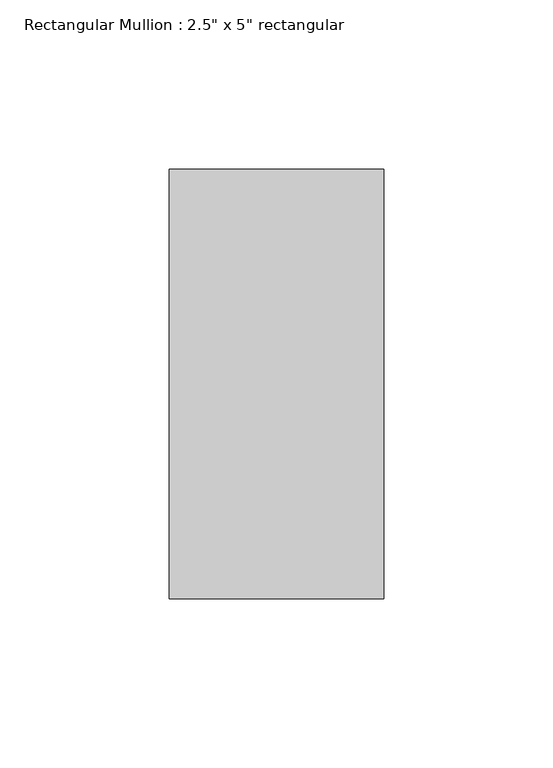
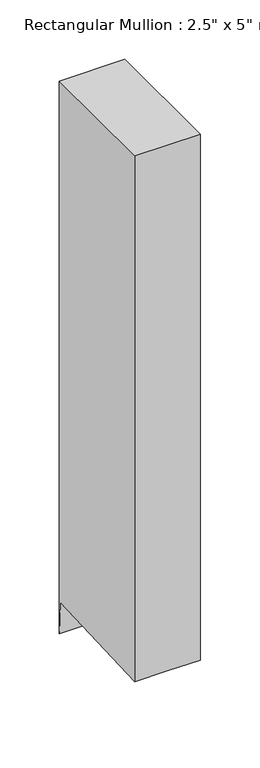
"""IFC4 building model written with IfcOpenShell, lengths in millimetres: member geometry."""

import ifcopenshell
import ifcopenshell.guid

model = None  # the IFC model being written
_history = None  # IfcOwnerHistory: only IFC2X3 demands one
_inside = {}  # id of a spatial element -> (the spatial element, [elements in it])
_under = {}  # id of a project, library or spatial element -> (it, [spatial elements below it])
_declared = {}  # id of a project -> (the project, [libraries it declares])
_typed = {}  # id of a type object -> (the type object, [elements of that type])
_made_of = {}  # id of a material, layer set ... -> (it, [elements and type objects made of it])


def new_model(schema):
    """Start an empty IFC model of exactly this schema.

    Asked for "IFC4X3", IfcOpenShell would pick the latest addendum, in which some entities
    have other attributes; the version numbers below select the first issue.
    IFC2X3 requires an IfcOwnerHistory on every rooted entity: one is made here for all.
    """
    global model, _history
    if schema == "IFC4X3":
        model = ifcopenshell.file(schema_version=(4, 3, 0, 0))
    else:
        model = ifcopenshell.file(schema=schema)
    _inside.clear()
    _under.clear()
    _declared.clear()
    _typed.clear()
    _made_of.clear()
    _history = None
    if model.schema == "IFC2X3":
        org = make("IfcOrganization", Name="unknown")
        user = make(
            "IfcPersonAndOrganization",
            ThePerson=make("IfcPerson", FamilyName="unknown"),
            TheOrganization=org,
        )
        app = make(
            "IfcApplication",
            ApplicationDeveloper=org,
            Version="unknown",
            ApplicationFullName="unknown",
            ApplicationIdentifier="unknown",
        )
        _history = make(
            "IfcOwnerHistory",
            OwningUser=user,
            OwningApplication=app,
            ChangeAction="ADDED",
            CreationDate=0,
        )
    return model


def make(cls, **values):
    """One entity of the class cls with the attributes given. An attribute that is None is left unset."""
    return model.create_entity(
        cls, **{name: value for name, value in values.items() if value is not None}
    )


def rooted(cls, **values):
    """An entity with a GlobalId (a new one), such as an element, a storey or a relation."""
    return make(cls, GlobalId=ifcopenshell.guid.new(), OwnerHistory=_history, **values)


def si_unit(unit_type, name, prefix=None):
    """IfcSIUnit, for example si_unit("LENGTHUNIT", "METRE", prefix="MILLI")."""
    return make("IfcSIUnit", UnitType=unit_type, Prefix=prefix, Name=name)


def assignment(units):
    """IfcUnitAssignment: the units of a project."""
    return None if units is None else make("IfcUnitAssignment", Units=units)


def point(xyz):
    """IfcCartesianPoint."""
    return None if xyz is None else make("IfcCartesianPoint", Coordinates=xyz)


def direction(xyz):
    """IfcDirection."""
    return None if xyz is None else make("IfcDirection", DirectionRatios=xyz)


def frame(location, z_axis=None, x_axis=None):
    """IfcAxis2Placement3D, a coordinate frame: its origin and axes. An axis left out is left unset."""
    return make(
        "IfcAxis2Placement3D",
        Location=point(location),
        Axis=direction(z_axis),
        RefDirection=direction(x_axis),
    )


def origin():
    """The frame at (0, 0, 0) with its axes left unset."""
    return frame((0.0, 0.0, 0.0))


def place(relative_to, where):
    """IfcLocalPlacement: puts the frame where relative to a parent placement (None: the world)."""
    return make(
        "IfcLocalPlacement", PlacementRelTo=relative_to, RelativePlacement=where
    )


def context(
    kind, dimensions, precision=None, world=None, true_north=None, identifier=None
):
    """IfcGeometricRepresentationContext, for example the 3D "Model" context."""
    return make(
        "IfcGeometricRepresentationContext",
        ContextIdentifier=identifier,
        ContextType=kind,
        CoordinateSpaceDimension=dimensions,
        Precision=precision,
        WorldCoordinateSystem=world,
        TrueNorth=true_north,
    )


def project(units=None, contexts=None):
    """IfcProject with its units and contexts."""
    return rooted(
        "IfcProject",
        Name="project",
        RepresentationContexts=contexts,
        UnitsInContext=assignment(units),
    )


def spatial(cls, under=None, at=None, **own):
    """A site, building, storey or space (cls), placed at a placement, below another one or the project."""
    s = rooted(cls, ObjectPlacement=at, **own)
    if under is not None:
        _under.setdefault(under.id(), (under, []))[1].append(s)
    return s


def faces_of(points, faces, orient=None, outer=None):
    """IfcFace entities. A face is a list of loops; a loop is a list of indices into points, from 0.

    orient and outer hold one flag for each loop. By default every Orientation is true, the
    first loop of a face is its IfcFaceOuterBound and the others are IfcFaceBound.
    """
    made = []
    for i, loops in enumerate(faces):
        bounds = []
        for j, loop in enumerate(loops):
            is_outer = j == 0 if outer is None else outer[i][j]
            bounds.append(
                make(
                    "IfcFaceOuterBound" if is_outer else "IfcFaceBound",
                    Bound=make("IfcPolyLoop", Polygon=[points[k] for k in loop]),
                    Orientation=True if orient is None else orient[i][j],
                )
            )
        made.append(make("IfcFace", Bounds=bounds))
    return made


def faceted_brep(points, faces, orient=None, outer=None, voids=None):
    """IfcFacetedBrep: a solid bounded by flat faces; with voids (closed shells), ...WithVoids."""
    shared = [point(p) for p in points]
    hull = make("IfcClosedShell", CfsFaces=faces_of(shared, faces, orient, outer))
    if voids is None:
        return make("IfcFacetedBrep", Outer=hull)
    return make(
        "IfcFacetedBrepWithVoids",
        Outer=hull,
        Voids=[
            make(cls, CfsFaces=faces_of(shared, fs, o, b)) for cls, fs, o, b in voids
        ],
    )


def shape(context_of_items, identifier, shape_type, items):
    """IfcShapeRepresentation: the items that make up one representation, for example the "Body"."""
    return make(
        "IfcShapeRepresentation",
        ContextOfItems=context_of_items,
        RepresentationIdentifier=identifier,
        RepresentationType=shape_type,
        Items=items,
    )


def source(mapping_origin, context_of_items, identifier, shape_type, items):
    """IfcRepresentationMap: a shape defined once, which mapped items show again and again."""
    return make(
        "IfcRepresentationMap",
        MappingOrigin=mapping_origin,
        MappedRepresentation=shape(context_of_items, identifier, shape_type, items),
    )


def transform(
    local_origin,
    x_axis=None,
    y_axis=None,
    z_axis=None,
    scale=None,
    scale2=None,
    scale3=None,
    uniform=True,
):
    """IfcCartesianTransformationOperator3D, or its non-uniform kind. x_axis, y_axis, z_axis: its Axis1, 2, 3."""
    if uniform:
        return make(
            "IfcCartesianTransformationOperator3D",
            Axis1=direction(x_axis),
            Axis2=direction(y_axis),
            LocalOrigin=point(local_origin),
            Scale=scale,
            Axis3=direction(z_axis),
        )
    return make(
        "IfcCartesianTransformationOperator3DnonUniform",
        Axis1=direction(x_axis),
        Axis2=direction(y_axis),
        LocalOrigin=point(local_origin),
        Scale=scale,
        Axis3=direction(z_axis),
        Scale2=scale2,
        Scale3=scale3,
    )


def mapped(mapping_source, mapping_target):
    """IfcMappedItem: shows the shape of a source again, moved by a transform."""
    return make(
        "IfcMappedItem", MappingSource=mapping_source, MappingTarget=mapping_target
    )


def made_of(thing, what):
    """Note that an element or type object is made of a material, layer set ...; save() writes the relation."""
    if what is not None:
        _made_of.setdefault(what.id(), (what, []))[1].append(thing)
    return thing


def element(
    cls,
    number,
    at=None,
    inside=None,
    cuts=None,
    type_object=None,
    material=None,
    context=None,
    identifier="Body",
    shape_type=None,
    held_by="IfcProductDefinitionShape",
    body=None,
    shapes=None,
    **own,
):
    """One element of the class cls, such as IfcWall. Its Tag is "e" and its number.

    at: its placement. inside: the storey or other place that contains it. cuts: it is an
    opening in that element (IfcRelVoidsElement). A single representation is given by context,
    identifier, shape_type and body (its items); several are given by shapes. held_by: the class
    of the entity that holds the representations. save() writes the other relations.
    """
    e = rooted(cls, Tag="e%d" % number, ObjectPlacement=at, **own)
    if body is not None:
        shapes = [shape(context, identifier, shape_type, body)]
    if shapes is not None:
        e.Representation = make(held_by, Representations=shapes)
    if inside is not None:
        _inside.setdefault(inside.id(), (inside, []))[1].append(e)
    if cuts is not None:
        rooted(
            "IfcRelVoidsElement", RelatingBuildingElement=cuts, RelatedOpeningElement=e
        )
    if type_object is not None:
        _typed.setdefault(type_object.id(), (type_object, []))[1].append(e)
    return made_of(e, material)


def aggregate(whole, parts):
    """IfcRelAggregates: a whole, such as a stair, and the parts it consists of."""
    return rooted("IfcRelAggregates", RelatingObject=whole, RelatedObjects=parts)


def save(model, path):
    """Write the relations noted so far, then the file.

    IfcRelAggregates (storeys below a building ...), IfcRelContainedInSpatialStructure (elements
    in a storey), IfcRelDefinesByType, IfcRelAssociatesMaterial and IfcRelDeclares: one each for
    every whole, place, type object, material and project.
    """
    for whole, parts in _under.values():
        aggregate(whole, parts)
    for where, things in _inside.values():
        rooted(
            "IfcRelContainedInSpatialStructure",
            RelatedElements=things,
            RelatingStructure=where,
        )
    for kind, things in _typed.values():
        rooted("IfcRelDefinesByType", RelatedObjects=things, RelatingType=kind)
    for what, things in _made_of.values():
        rooted("IfcRelAssociatesMaterial", RelatedObjects=things, RelatingMaterial=what)
    for by, libraries in _declared.values():
        rooted("IfcRelDeclares", RelatingContext=by, RelatedDefinitions=libraries)
    model.write(path)


def member_d4789dbb(model_context):
    return source(origin(), model_context, "Body", "Brep", [
        faceted_brep([(31.75, 63.5, 0.0), (-31.75, 63.5, 0.0), (-31.75, -63.5, 0.0), (31.75, -63.5, 0.0), (31.75, 63.5, -568.018324), (0.0, 63.5, -568.018324), (-31.75, 63.5, -568.018324), (-31.75, 62.0828234, -534.9390623), (-31.75, -63.5, -540.3192622), (0.0, -63.5, -540.3192622), (31.75, -63.5, -540.3192622), (31.75, 62.0828234, -534.9390623), (0.0, 62.0828234, -534.9390623)], [[[0, 1, 2, 3]], [[1, 0, 4, 5, 6]], [[2, 1, 6, 7, 8]], [[3, 2, 8, 9, 10]], [[0, 3, 10, 11, 4]], [[4, 11, 12, 5]], [[11, 10, 9, 12]], [[9, 8, 7, 12]], [[7, 6, 5, 12]]]),
    ])


if __name__ == "__main__":
    model = new_model("IFC4")
    model_context = context("Model", 3, world=origin())
    ifc_project = project(units=[si_unit("LENGTHUNIT", "METRE", prefix="MILLI")], contexts=[model_context])
    site = spatial("IfcSite", under=ifc_project)
    building = spatial("IfcBuilding", under=site)
    placement = place(None, origin())
    member_shape = member_d4789dbb(model_context)
    element("IfcMember", 1, ObjectType="Rectangular Mullion : 2.5\" x 5\" rectangular", at=placement, inside=building, context=model_context, shape_type="MappedRepresentation", body=[
        mapped(member_shape, transform((0.0, 0.0, 0.0), x_axis=(1.0, 0.0, 0.0), y_axis=(0.0, 1.0, 0.0), z_axis=(0.0, 0.0, 1.0))),
    ])
    save(model, "model.ifc")

# Revit data of these elements
# Type "Rectangular Mullion : 2.5\" x 5\" rectangular"
#   built-in parameter 1007304 = 0.416667 (stored number, unit not read)
#   built-in parameter 1007301 = 0.104167 (stored number, unit not read)
#   built-in parameter 1007300 = 0.104167 (stored number, unit not read)
# Element 1 (IfcMember, "Rectangular Mullion : 2.5\" x 5\" rectangular")
#   Materials on its faces: "Metal - Aluminum"
# Materials
#   "Metal - Aluminum": class "Metal", colour RGB 247 247 247, transparency 0, Cost = 0
